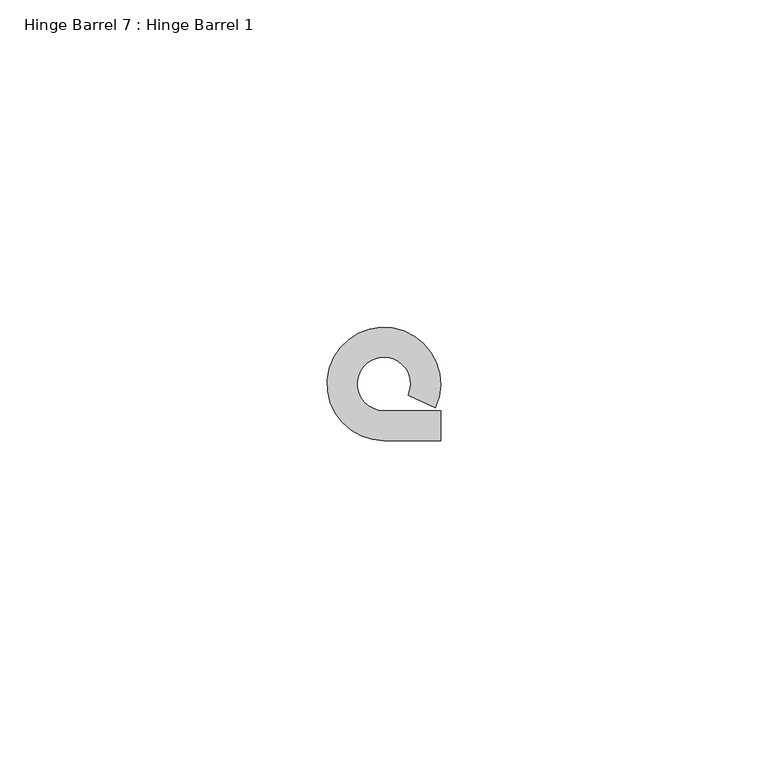
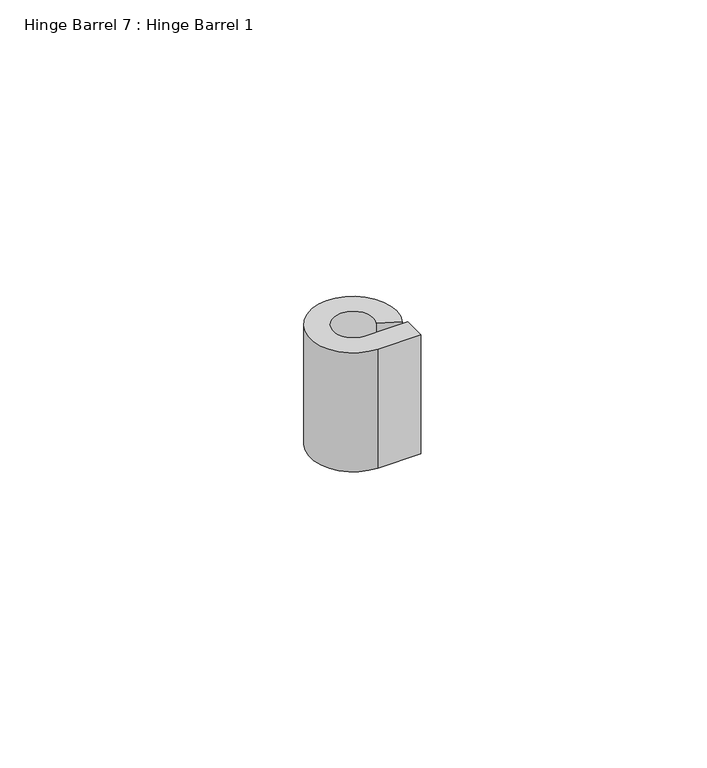
"""IFC4 building model written with IfcOpenShell, lengths in millimetres: proxy geometry, Hinge Barrel 7 : Hinge Barrel 1."""

from ifc_helpers import new_model, si_unit, point, frame, frame_2d, origin, place, context, project, spatial, polyline, circle_curve, trimmed, segment, composite_curve, outline, extrude, source, transform, mapped, element, save


def hinge_barrel_7_hinge_barrel_1_4fbccd9d(model_context):
    return source(origin(), model_context, "Body", "SweptSolid", [
        extrude(outline(composite_curve([segment(polyline([(587323.2214739, -531780.6943841), (587327.7934739, -531780.6943841), (587327.7934739, -531785.2584466), (587319.1320739, -531785.2584466)]), True, "CONTINUOUS"), segment(trimmed(circle_curve(frame_2d((587319.1320739, -531776.6049841)), 8.6534625), [point((587319.1320739, -531785.2584466))], [point((587326.986084, -531780.2377433))], False, "CARTESIAN"), True, "CONTINUOUS"), segment(polyline([(587326.986084, -531780.2377433), (587322.8436736, -531778.321731)]), True, "CONTINUOUS"), segment(trimmed(circle_curve(frame_2d((587319.1320739, -531776.6049841)), 4.0894), [point((587322.8436736, -531778.321731))], [point((587319.1320739, -531780.6943841))], True, "CARTESIAN"), True, "CONTINUOUS"), segment(polyline([(587319.1320739, -531780.6943841), (587323.2214739, -531780.6943841)]), True, "CONTINUOUS")], self_intersect=False)), frame((0.0, 0.0, 1936.75), z_axis=(0.0, 0.0, 1.0), x_axis=(1.0, 0.0, 0.0)), (0.0, 0.0, 1.0), 25.4),
    ])


if __name__ == "__main__":
    model = new_model("IFC4")
    model_context = context("Model", 3, world=origin())
    ifc_project = project(units=[si_unit("LENGTHUNIT", "METRE", prefix="MILLI")], contexts=[model_context])
    site = spatial("IfcSite", under=ifc_project)
    building = spatial("IfcBuilding", under=site)
    placement = place(None, origin())
    hinge_barrel_7_hinge_barrel_1_shape = hinge_barrel_7_hinge_barrel_1_4fbccd9d(model_context)
    element("IfcBuildingElementProxy", 1, Name="Hinge Barrel 7 : Hinge Barrel 1", ObjectType="Hinge Barrel 7 : Hinge Barrel 1", at=placement, inside=building, context=model_context, shape_type="MappedRepresentation", body=[
        mapped(hinge_barrel_7_hinge_barrel_1_shape, transform((0.0, 0.0, 0.0), x_axis=(1.0, 0.0, 0.0), y_axis=(0.0, 1.0, 0.0), z_axis=(0.0, 0.0, 1.0))),
    ])
    save(model, "model.ifc")

# Revit data of these elements
# Element 1 (IfcBuildingElementProxy, "Hinge Barrel 7 : Hinge Barrel 1")
#   Materials on its faces: "6\"X6\" WELD-ON STL BUTT HINGE"
# Materials
#   "6\"X6\" WELD-ON STL BUTT HINGE": class "Metal", colour RGB 189 187 185, transparency 0, Description = "Carbon steel", Cost = 0
